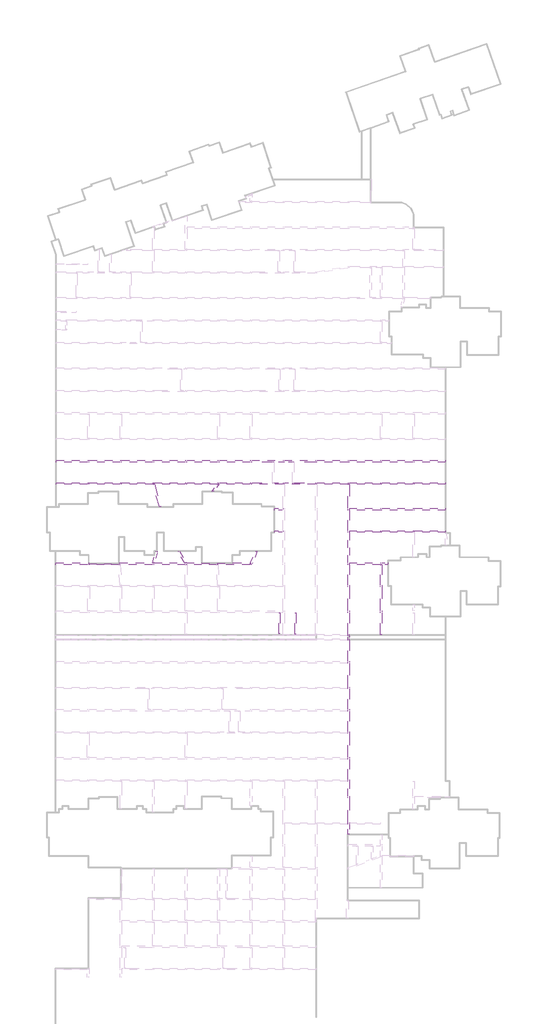
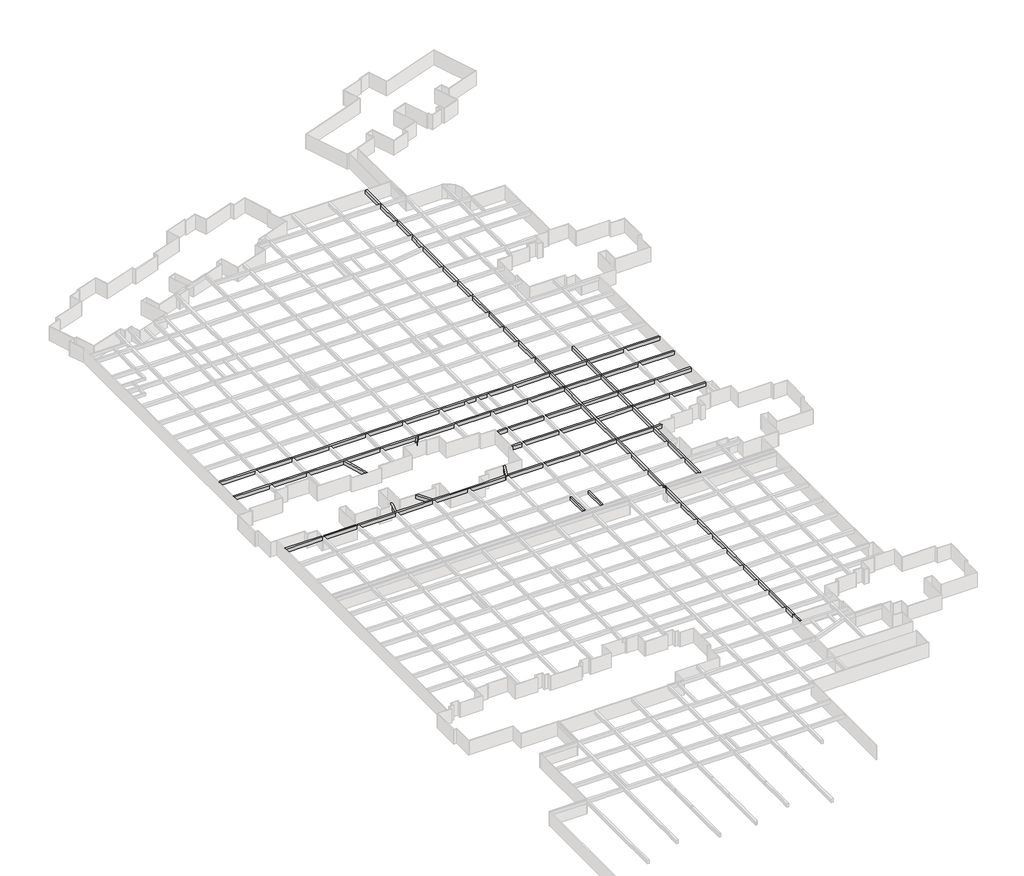
# One storey, part 11 of 14: 17 beams.
"""IFC4 building model written with IfcOpenShell, lengths in millimetres."""

from ifc_helpers import new_model, si_unit, frame, origin, place, context, project, spatial, polyline, outline, extrude, faceted_brep, element, save

model = new_model("IFC4")

# Units and contexts
model_context = context("Model", 3, world=origin())
ifc_project = project(units=[si_unit("LENGTHUNIT", "METRE", prefix="MILLI")], contexts=[model_context])

# Site, building, storey
site = spatial("IfcSite", under=ifc_project)
building = spatial("IfcBuilding", under=site)
storey = spatial("IfcBuildingStorey", under=building, Name="户型图", Elevation=0.0)

# Beams
placement = place(None, origin())
element("IfcBeam", 1, ObjectType="混凝土 - 矩形梁 : KL_beam", at=placement, inside=storey, context=model_context, shape_type="Brep", body=[
    faceted_brep([(-594019.2557706, -85259.4327531, 3300.0), (-594019.2557706, -85659.4327531, 3300.0), (-586267.6529954, -85659.4327531, 3300.0), (-585867.6529954, -85659.4327531, 3300.0), (-578267.6529954, -85659.4327531, 3300.0), (-577867.6529954, -85659.4327531, 3300.0), (-570267.6529954, -85659.4327531, 3300.0), (-569867.6529954, -85659.4327531, 3300.0), (-562267.6529954, -85659.4327531, 3300.0), (-561867.6529954, -85659.4327531, 3300.0), (-554267.6529954, -85659.4327531, 3300.0), (-553867.6529954, -85659.4327531, 3300.0), (-546267.6529954, -85659.4327531, 3300.0), (-545867.6529954, -85659.4327531, 3300.0), (-540767.6529954, -85659.4327531, 3300.0), (-540467.6529954, -85659.4327531, 3300.0), (-538267.6529954, -85659.4327531, 3300.0), (-537867.6529954, -85659.4327531, 3300.0), (-535867.6529954, -85659.4327531, 3300.0), (-535567.6529954, -85659.4327531, 3300.0), (-530267.6529954, -85659.4327531, 3300.0), (-529867.6529954, -85659.4327531, 3300.0), (-522267.6529954, -85659.4327531, 3300.0), (-521867.6529954, -85659.4327531, 3300.0), (-514267.6529954, -85659.4327531, 3300.0), (-513867.6529954, -85659.4327531, 3300.0), (-506267.6529954, -85659.4327531, 3300.0), (-505867.6529954, -85659.4327531, 3300.0), (-498277.6529954, -85659.4327531, 3300.0), (-498277.6529954, -85259.4327531, 3300.0), (-505867.6529954, -85259.4327531, 3300.0), (-506267.6529954, -85259.4327531, 3300.0), (-513867.6529954, -85259.4327531, 3300.0), (-514267.6529954, -85259.4327531, 3300.0), (-521867.6529954, -85259.4327531, 3300.0), (-522267.6529954, -85259.4327531, 3300.0), (-529867.6529954, -85259.4327531, 3300.0), (-530267.6529954, -85259.4327531, 3300.0), (-537867.6529954, -85259.4327531, 3300.0), (-538267.6529954, -85259.4327531, 3300.0), (-545867.6529954, -85259.4327531, 3300.0), (-546267.6529954, -85259.4327531, 3300.0), (-553867.6529954, -85259.4327531, 3300.0), (-554267.6529954, -85259.4327531, 3300.0), (-561867.6529954, -85259.4327531, 3300.0), (-562267.6529954, -85259.4327531, 3300.0), (-569867.6529954, -85259.4327531, 3300.0), (-570267.6529954, -85259.4327531, 3300.0), (-577867.6529954, -85259.4327531, 3300.0), (-578267.6529954, -85259.4327531, 3300.0), (-585867.6529954, -85259.4327531, 3300.0), (-586267.6529954, -85259.4327531, 3300.0), (-594019.2557706, -85659.4327531, 2500.0), (-586267.6529954, -85659.4327531, 2500.0), (-585867.6529954, -85659.4327531, 2500.0), (-578267.6529954, -85659.4327531, 2500.0), (-577867.6529954, -85659.4327531, 2500.0), (-570267.6529954, -85659.4327531, 2500.0), (-569867.6529954, -85659.4327531, 2500.0), (-562267.6529954, -85659.4327531, 2500.0), (-561867.6529954, -85659.4327531, 2500.0), (-554267.6529954, -85659.4327531, 2500.0), (-553867.6529954, -85659.4327531, 2500.0), (-546267.6529954, -85659.4327531, 2500.0), (-545867.6529954, -85659.4327531, 2500.0), (-538267.6529954, -85659.4327531, 2500.0), (-537867.6529954, -85659.4327531, 2500.0), (-530267.6529954, -85659.4327531, 2500.0), (-529867.6529954, -85659.4327531, 2500.0), (-522267.6529954, -85659.4327531, 2500.0), (-521867.6529954, -85659.4327531, 2500.0), (-514267.6529954, -85659.4327531, 2500.0), (-513867.6529954, -85659.4327531, 2500.0), (-506267.6529954, -85659.4327531, 2500.0), (-505867.6529954, -85659.4327531, 2500.0), (-498277.6529954, -85659.4327531, 2500.0), (-594019.2557706, -85259.4327531, 2500.0), (-586267.6529954, -85259.4327531, 2500.0), (-585867.6529954, -85259.4327531, 2500.0), (-578267.6529954, -85259.4327531, 2500.0), (-577867.6529954, -85259.4327531, 2500.0), (-570267.6529954, -85259.4327531, 2500.0), (-569867.6529954, -85259.4327531, 2500.0), (-562267.6529954, -85259.4327531, 2500.0), (-561867.6529954, -85259.4327531, 2500.0), (-554267.6529954, -85259.4327531, 2500.0), (-553867.6529954, -85259.4327531, 2500.0), (-546267.6529954, -85259.4327531, 2500.0), (-545867.6529954, -85259.4327531, 2500.0), (-538267.6529954, -85259.4327531, 2500.0), (-537867.6529954, -85259.4327531, 2500.0), (-530267.6529954, -85259.4327531, 2500.0), (-529867.6529954, -85259.4327531, 2500.0), (-522267.6529954, -85259.4327531, 2500.0), (-521867.6529954, -85259.4327531, 2500.0), (-514267.6529954, -85259.4327531, 2500.0), (-513867.6529954, -85259.4327531, 2500.0), (-506267.6529954, -85259.4327531, 2500.0), (-505867.6529954, -85259.4327531, 2500.0), (-498277.6529954, -85259.4327531, 2500.0)], [[[0, 1, 2, 3, 4, 5, 6, 7, 8, 9, 10, 11, 12, 13, 14, 15, 16, 17, 18, 19, 20, 21, 22, 23, 24, 25, 26, 27, 28, 29, 30, 31, 32, 33, 34, 35, 36, 37, 38, 39, 40, 41, 42, 43, 44, 45, 46, 47, 48, 49, 50, 51]], [[1, 52, 53, 54, 55, 56, 57, 58, 59, 60, 61, 62, 63, 64, 65, 66, 67, 68, 69, 70, 71, 72, 73, 74, 75, 28, 27, 26, 25, 24, 23, 22, 21, 20, 19, 18, 17, 16, 15, 14, 13, 12, 11, 10, 9, 8, 7, 6, 5, 4, 3, 2]], [[52, 76, 77, 78, 79, 80, 81, 82, 83, 84, 85, 86, 87, 88, 89, 90, 91, 92, 93, 94, 95, 96, 97, 98, 99, 75, 74, 73, 72, 71, 70, 69, 68, 67, 66, 65, 64, 63, 62, 61, 60, 59, 58, 57, 56, 55, 54, 53]], [[76, 0, 51, 50, 49, 48, 47, 46, 45, 44, 43, 42, 41, 40, 39, 38, 37, 36, 35, 34, 33, 32, 31, 30, 29, 99, 98, 97, 96, 95, 94, 93, 92, 91, 90, 89, 88, 87, 86, 85, 84, 83, 82, 81, 80, 79, 78, 77]], [[1, 0, 76, 52]], [[29, 28, 75, 99]]]),
])
element("IfcBeam", 2, ObjectType="混凝土 - 矩形梁 : KL_beam", at=placement, inside=storey, context=model_context, shape_type="Brep", body=[
    faceted_brep([(-594019.2557706, -90759.4327531, 3300.0), (-594019.2557706, -91159.4327531, 3300.0), (-586267.6529954, -91159.4327531, 3300.0), (-585867.6529954, -91159.4327531, 3300.0), (-578267.6529954, -91159.4327531, 3300.0), (-577867.6529954, -91159.4327531, 3300.0), (-570217.8756354, -91159.4327531, 3300.0), (-569801.3815466, -91159.4327531, 3300.0), (-562267.6529954, -91159.4327531, 3300.0), (-561867.6529954, -91159.4327531, 3300.0), (-554452.1630717, -91159.4327531, 3300.0), (-553963.8532362, -91159.4327531, 3300.0), (-546267.6529954, -91159.4327531, 3300.0), (-545867.6529954, -91159.4327531, 3300.0), (-538267.6529954, -91159.4327531, 3300.0), (-537867.6529954, -91159.4327531, 3300.0), (-530267.6529954, -91159.4327531, 3300.0), (-529867.6529954, -91159.4327531, 3300.0), (-522267.6529954, -91159.4327531, 3300.0), (-521867.6529954, -91159.4327531, 3300.0), (-514267.6529954, -91159.4327531, 3300.0), (-513867.6529954, -91159.4327531, 3300.0), (-506267.6529954, -91159.4327531, 3300.0), (-505867.6529954, -91159.4327531, 3300.0), (-498277.6529954, -91159.4327531, 3300.0), (-498277.6529954, -90759.4327531, 3300.0), (-505867.6529954, -90759.4327531, 3300.0), (-506267.6529954, -90759.4327531, 3300.0), (-513867.6529954, -90759.4327531, 3300.0), (-514267.6529954, -90759.4327531, 3300.0), (-521867.6529954, -90759.4327531, 3300.0), (-522267.6529954, -90759.4327531, 3300.0), (-529867.6529954, -90759.4327531, 3300.0), (-530267.6529954, -90759.4327531, 3300.0), (-535567.6529954, -90759.4327531, 3300.0), (-535867.6529954, -90759.4327531, 3300.0), (-537867.6529954, -90759.4327531, 3300.0), (-538267.6529954, -90759.4327531, 3300.0), (-540467.6529954, -90759.4327531, 3300.0), (-540767.6529954, -90759.4327531, 3300.0), (-545867.6529954, -90759.4327531, 3300.0), (-546267.6529954, -90759.4327531, 3300.0), (-553867.6529954, -90759.4327531, 3300.0), (-554267.6529954, -90759.4327531, 3300.0), (-561867.6529954, -90759.4327531, 3300.0), (-562267.6529954, -90759.4327531, 3300.0), (-569867.6529954, -90759.4327531, 3300.0), (-570267.6529954, -90759.4327531, 3300.0), (-577867.6529954, -90759.4327531, 3300.0), (-578267.6529954, -90759.4327531, 3300.0), (-585867.6529954, -90759.4327531, 3300.0), (-586267.6529954, -90759.4327531, 3300.0), (-594019.2557706, -90759.4327531, 2500.0), (-498277.6529954, -90759.4327531, 2500.0), (-505867.6529954, -90759.4327531, 2500.0), (-506267.6529954, -90759.4327531, 2500.0), (-513867.6529954, -90759.4327531, 2500.0), (-514267.6529954, -90759.4327531, 2500.0), (-521867.6529954, -90759.4327531, 2500.0), (-522267.6529954, -90759.4327531, 2500.0), (-529867.6529954, -90759.4327531, 2500.0), (-530267.6529954, -90759.4327531, 2500.0), (-537867.6529954, -90759.4327531, 2500.0), (-538267.6529954, -90759.4327531, 2500.0), (-545867.6529954, -90759.4327531, 2500.0), (-546267.6529954, -90759.4327531, 2500.0), (-553867.6529954, -90759.4327531, 2500.0), (-554267.6529954, -90759.4327531, 2500.0), (-561867.6529954, -90759.4327531, 2500.0), (-562267.6529954, -90759.4327531, 2500.0), (-569867.6529954, -90759.4327531, 2500.0), (-570267.6529954, -90759.4327531, 2500.0), (-577867.6529954, -90759.4327531, 2500.0), (-578267.6529954, -90759.4327531, 2500.0), (-585867.6529954, -90759.4327531, 2500.0), (-586267.6529954, -90759.4327531, 2500.0), (-594019.2557706, -91159.4327531, 2500.0), (-498277.6529954, -91159.4327531, 2500.0), (-505867.6529954, -91159.4327531, 2500.0), (-506267.6529954, -91159.4327531, 2500.0), (-513867.6529954, -91159.4327531, 2500.0), (-514267.6529954, -91159.4327531, 2500.0), (-521867.6529954, -91159.4327531, 2500.0), (-522267.6529954, -91159.4327531, 2500.0), (-529867.6529954, -91159.4327531, 2500.0), (-530267.6529954, -91159.4327531, 2500.0), (-537867.6529954, -91159.4327531, 2500.0), (-538267.6529954, -91159.4327531, 2500.0), (-545867.6529954, -91159.4327531, 2500.0), (-546267.6529954, -91159.4327531, 2500.0), (-553963.8532362, -91159.4327531, 2500.0), (-554452.1630717, -91159.4327531, 2500.0), (-561867.6529954, -91159.4327531, 2500.0), (-562267.6529954, -91159.4327531, 2500.0), (-569801.3815466, -91159.4327531, 2500.0), (-570217.8756354, -91159.4327531, 2500.0), (-577867.6529954, -91159.4327531, 2500.0), (-578267.6529954, -91159.4327531, 2500.0), (-585867.6529954, -91159.4327531, 2500.0), (-586267.6529954, -91159.4327531, 2500.0)], [[[0, 1, 2, 3, 4, 5, 6, 7, 8, 9, 10, 11, 12, 13, 14, 15, 16, 17, 18, 19, 20, 21, 22, 23, 24, 25, 26, 27, 28, 29, 30, 31, 32, 33, 34, 35, 36, 37, 38, 39, 40, 41, 42, 43, 44, 45, 46, 47, 48, 49, 50, 51]], [[52, 0, 51, 50, 49, 48, 47, 46, 45, 44, 43, 42, 41, 40, 39, 38, 37, 36, 35, 34, 33, 32, 31, 30, 29, 28, 27, 26, 25, 53, 54, 55, 56, 57, 58, 59, 60, 61, 62, 63, 64, 65, 66, 67, 68, 69, 70, 71, 72, 73, 74, 75]], [[76, 52, 75, 74, 73, 72, 71, 70, 69, 68, 67, 66, 65, 64, 63, 62, 61, 60, 59, 58, 57, 56, 55, 54, 53, 77, 78, 79, 80, 81, 82, 83, 84, 85, 86, 87, 88, 89, 90, 91, 92, 93, 94, 95, 96, 97, 98, 99]], [[1, 76, 99, 98, 97, 96, 95, 94, 93, 92, 91, 90, 89, 88, 87, 86, 85, 84, 83, 82, 81, 80, 79, 78, 77, 24, 23, 22, 21, 20, 19, 18, 17, 16, 15, 14, 13, 12, 11, 10, 9, 8, 7, 6, 5, 4, 3, 2]], [[1, 0, 52, 76]], [[25, 24, 77, 53]]]),
])
element("IfcBeam", 3, ObjectType="混凝土 - 矩形梁 : KL_beam", at=placement, inside=storey, context=model_context, shape_type="SweptSolid", body=[
    extrude(outline(polyline([(-568206.7540557, -96655.8355445), (-568623.2481445, -96655.8355445), (-570217.8756354, -91159.4327531), (-569801.3815466, -91159.4327531), (-568206.7540557, -96655.8355445)])), frame((0.0, 0.0, 2500.0), z_axis=(0.0, 0.0, 1.0), x_axis=(1.0, 0.0, 0.0)), (0.0, 0.0, 1.0), 800.0),
])
element("IfcBeam", 4, ObjectType="混凝土 - 矩形梁 : KL_beam", at=placement, inside=storey, context=model_context, shape_type="Brep", body=[
    faceted_brep([(-521867.6529954, -16219.4327531, 3300.0), (-522267.6529954, -16219.4327531, 3300.0), (-522267.6529954, -21559.4327531, 3300.0), (-521867.6529954, -21559.4327531, 3300.0), (-522267.6529954, -16219.4327531, 2500.0), (-522267.6529954, -21559.4327531, 2500.0), (-521867.6529954, -16219.4327531, 2500.0), (-521867.6529954, -21559.4327531, 2500.0)], [[[0, 1, 2, 3]], [[1, 4, 5, 2]], [[4, 6, 7, 5]], [[6, 0, 3, 7]], [[1, 0, 6, 4]], [[3, 2, 5, 7]]]),
    faceted_brep([(-521867.6529954, -177127.2416788, 3300.0), (-522267.6529954, -177127.2416788, 3300.0), (-522267.6529954, -177127.2416788, 2500.0), (-521867.6529954, -177127.2416788, 2500.0), (-522267.6529954, -91159.4327531, 3300.0), (-521867.6529954, -91159.4327531, 3300.0), (-521867.6529954, -91159.4327531, 2500.0), (-522267.6529954, -91159.4327531, 2500.0), (-521952.6098527, -128219.4327532, 2500.0), (-521952.6098527, -128219.4327532, 3300.0), (-521867.6529954, -128219.4327532, 3300.0), (-521867.6529954, -128219.4327532, 2500.0), (-521952.6098527, -128099.4327532, 3300.0), (-521952.6098527, -128099.4327532, 2500.0), (-521867.6529954, -128099.4327532, 2500.0), (-521867.6529954, -128099.4327532, 3300.0), (-521952.6098527, -129174.4327531, 3300.0), (-521952.6098527, -129174.4327531, 2500.0), (-521867.6529954, -129174.4327531, 2500.0), (-521867.6529954, -129174.4327531, 3300.0), (-521952.6098527, -129294.4327531, 2500.0), (-521952.6098527, -129294.4327531, 3300.0), (-521867.6529954, -129294.4327531, 3300.0), (-521867.6529954, -129294.4327531, 2500.0), (-521867.6529954, -174657.5200046, 3300.0), (-521867.6529954, -174257.5200046, 3300.0), (-521867.6529954, -168200.507479, 3300.0), (-521867.6529954, -167800.507479, 3300.0), (-521867.6529954, -164159.4327531, 3300.0), (-521867.6529954, -163759.4327531, 3300.0), (-521867.6529954, -158659.4327531, 3300.0), (-521867.6529954, -158259.4327531, 3300.0), (-521867.6529954, -152359.4327531, 3300.0), (-521867.6529954, -151959.4327531, 3300.0), (-521867.6529954, -146859.4327531, 3300.0), (-521867.6529954, -146459.4327531, 3300.0), (-521867.6529954, -141359.4327531, 3300.0), (-521867.6529954, -140959.4327531, 3300.0), (-521867.6529954, -135059.4327531, 3300.0), (-521867.6529954, -134659.4327531, 3300.0), (-521867.6529954, -129434.4327531, 3300.0), (-521867.6529954, -129034.4327531, 3300.0), (-521867.6529954, -128359.4327532, 3300.0), (-521867.6529954, -127959.4327532, 3300.0), (-521867.6529954, -122659.4327531, 3300.0), (-521867.6529954, -122259.4327531, 3300.0), (-521867.6529954, -116357.5126628, 3300.0), (-521867.6529954, -115957.5126628, 3300.0), (-521867.6529954, -110859.4327531, 3300.0), (-521867.6529954, -110459.4327531, 3300.0), (-521867.6529954, -102959.4327531, 3300.0), (-521867.6529954, -102559.4327531, 3300.0), (-521867.6529954, -97459.4327531, 3300.0), (-521867.6529954, -97059.4327531, 3300.0), (-522267.6529954, -97059.4327531, 3300.0), (-522267.6529954, -97459.4327531, 3300.0), (-522267.6529954, -102559.4327531, 3300.0), (-522267.6529954, -102959.4327531, 3300.0), (-522267.6529954, -110459.4327531, 3300.0), (-522267.6529954, -110859.4327531, 3300.0), (-522267.6529954, -115957.5126628, 3300.0), (-522267.6529954, -116357.5126628, 3300.0), (-522267.6529954, -122259.4327531, 3300.0), (-522267.6529954, -122659.4327531, 3300.0), (-522267.6529954, -127959.4327532, 3300.0), (-522267.6529954, -128359.4327532, 3300.0), (-522267.6529954, -129034.4327531, 3300.0), (-522267.6529954, -129434.4327531, 3300.0), (-522267.6529954, -134659.4327531, 3300.0), (-522267.6529954, -135059.4327531, 3300.0), (-522267.6529954, -140959.4327531, 3300.0), (-522267.6529954, -141359.4327531, 3300.0), (-522267.6529954, -146459.4327531, 3300.0), (-522267.6529954, -146859.4327531, 3300.0), (-522267.6529954, -151959.4327531, 3300.0), (-522267.6529954, -152359.4327531, 3300.0), (-522267.6529954, -158259.4327531, 3300.0), (-522267.6529954, -158659.4327531, 3300.0), (-522267.6529954, -163759.4327531, 3300.0), (-522267.6529954, -164159.4327531, 3300.0), (-522267.6529954, -167800.507479, 3300.0), (-522267.6529954, -168200.507479, 3300.0), (-522267.6529954, -174257.5200046, 3300.0), (-522267.6529954, -174657.5200046, 3300.0), (-522267.6529954, -97059.4327531, 2500.0), (-522267.6529954, -97459.4327531, 2500.0), (-522267.6529954, -102559.4327531, 2500.0), (-522267.6529954, -102959.4327531, 2500.0), (-522267.6529954, -110459.4327531, 2500.0), (-522267.6529954, -110859.4327531, 2500.0), (-522267.6529954, -115957.5126628, 2500.0), (-522267.6529954, -116357.5126628, 2500.0), (-522267.6529954, -122259.4327531, 2500.0), (-522267.6529954, -122659.4327531, 2500.0), (-522267.6529954, -127959.4327532, 2500.0), (-522267.6529954, -128359.4327532, 2500.0), (-522267.6529954, -129034.4327531, 2500.0), (-522267.6529954, -129434.4327531, 2500.0), (-522267.6529954, -134659.4327531, 2500.0), (-522267.6529954, -135059.4327531, 2500.0), (-522267.6529954, -140959.4327531, 2500.0), (-522267.6529954, -141359.4327531, 2500.0), (-522267.6529954, -146459.4327531, 2500.0), (-522267.6529954, -146859.4327531, 2500.0), (-522267.6529954, -151959.4327531, 2500.0), (-522267.6529954, -152359.4327531, 2500.0), (-522267.6529954, -158259.4327531, 2500.0), (-522267.6529954, -158659.4327531, 2500.0), (-522267.6529954, -163759.4327531, 2500.0), (-522267.6529954, -164159.4327531, 2500.0), (-522267.6529954, -167800.507479, 2500.0), (-522267.6529954, -168200.507479, 2500.0), (-522267.6529954, -174257.5200046, 2500.0), (-522267.6529954, -174657.5200046, 2500.0), (-521867.6529954, -97059.4327531, 2500.0), (-521867.6529954, -97459.4327531, 2500.0), (-521867.6529954, -102559.4327531, 2500.0), (-521867.6529954, -102959.4327531, 2500.0), (-521867.6529954, -110459.4327531, 2500.0), (-521867.6529954, -110859.4327531, 2500.0), (-521867.6529954, -115957.5126628, 2500.0), (-521867.6529954, -116357.5126628, 2500.0), (-521867.6529954, -122259.4327531, 2500.0), (-521867.6529954, -122659.4327531, 2500.0), (-521867.6529954, -127959.4327532, 2500.0), (-521867.6529954, -128359.4327532, 2500.0), (-521867.6529954, -129034.4327531, 2500.0), (-521867.6529954, -129434.4327531, 2500.0), (-521867.6529954, -134659.4327531, 2500.0), (-521867.6529954, -135059.4327531, 2500.0), (-521867.6529954, -140959.4327531, 2500.0), (-521867.6529954, -141359.4327531, 2500.0), (-521867.6529954, -146459.4327531, 2500.0), (-521867.6529954, -146859.4327531, 2500.0), (-521867.6529954, -151959.4327531, 2500.0), (-521867.6529954, -152359.4327531, 2500.0), (-521867.6529954, -158259.4327531, 2500.0), (-521867.6529954, -158659.4327531, 2500.0), (-521867.6529954, -163759.4327531, 2500.0), (-521867.6529954, -164159.4327531, 2500.0), (-521867.6529954, -167800.507479, 2500.0), (-521867.6529954, -168200.507479, 2500.0), (-521867.6529954, -174257.5200046, 2500.0), (-521867.6529954, -174657.5200046, 2500.0)], [[[0, 1, 2, 3]], [[4, 5, 6, 7]], [[8, 9, 10, 11]], [[12, 13, 14, 15]], [[9, 8, 13, 12]], [[16, 17, 18, 19]], [[20, 21, 22, 23]], [[17, 16, 21, 20]], [[1, 0, 24, 25, 26, 27, 28, 29, 30, 31, 32, 33, 34, 35, 36, 37, 38, 39, 40, 22, 21, 16, 19, 41, 42, 10, 9, 12, 15, 43, 44, 45, 46, 47, 48, 49, 50, 51, 52, 53, 5, 4, 54, 55, 56, 57, 58, 59, 60, 61, 62, 63, 64, 65, 66, 67, 68, 69, 70, 71, 72, 73, 74, 75, 76, 77, 78, 79, 80, 81, 82, 83]], [[2, 1, 83, 82, 81, 80, 79, 78, 77, 76, 75, 74, 73, 72, 71, 70, 69, 68, 67, 66, 65, 64, 63, 62, 61, 60, 59, 58, 57, 56, 55, 54, 4, 7, 84, 85, 86, 87, 88, 89, 90, 91, 92, 93, 94, 95, 96, 97, 98, 99, 100, 101, 102, 103, 104, 105, 106, 107, 108, 109, 110, 111, 112, 113]], [[3, 2, 113, 112, 111, 110, 109, 108, 107, 106, 105, 104, 103, 102, 101, 100, 99, 98, 97, 96, 95, 94, 93, 92, 91, 90, 89, 88, 87, 86, 85, 84, 7, 6, 114, 115, 116, 117, 118, 119, 120, 121, 122, 123, 124, 14, 13, 8, 11, 125, 126, 18, 17, 20, 23, 127, 128, 129, 130, 131, 132, 133, 134, 135, 136, 137, 138, 139, 140, 141, 142, 143]], [[0, 3, 143, 142, 141, 140, 139, 138, 137, 136, 135, 134, 133, 132, 131, 130, 129, 128, 127, 23, 22, 40, 39, 38, 37, 36, 35, 34, 33, 32, 31, 30, 29, 28, 27, 26, 25, 24]], [[6, 5, 53, 52, 51, 50, 49, 48, 47, 46, 45, 44, 43, 15, 14, 124, 123, 122, 121, 120, 119, 118, 117, 116, 115, 114]], [[11, 10, 42, 41, 19, 18, 126, 125]]]),
    faceted_brep([(-522267.6529954, -33759.4327531, 3300.0), (-521867.6529954, -33759.4327531, 3300.0), (-521867.6529954, -33759.4327531, 2500.0), (-522267.6529954, -33759.4327531, 2500.0), (-521867.6529954, -45159.4327531, 3300.0), (-522267.6529954, -45159.4327531, 3300.0), (-522267.6529954, -45159.4327531, 2500.0), (-521867.6529954, -45159.4327531, 2500.0), (-522267.6529954, -37589.309334, 3300.0), (-522267.6529954, -37994.5561723, 3300.0), (-521867.6529954, -37959.4327532, 3300.0), (-521867.6529954, -37559.4327532, 3300.0), (-522267.6529954, -37589.309334, 2500.0), (-522267.6529954, -37994.5561723, 2500.0), (-521867.6529954, -37559.4327532, 2500.0), (-521867.6529954, -37959.4327532, 2500.0)], [[[0, 1, 2, 3]], [[4, 5, 6, 7]], [[1, 0, 8, 9, 5, 4, 10, 11]], [[0, 3, 12, 13, 6, 5, 9, 8]], [[3, 2, 14, 15, 7, 6, 13, 12]], [[2, 1, 11, 10, 4, 7, 15, 14]]]),
    faceted_brep([(-521867.6529954, -33359.4327531, 3300.0), (-522267.6529954, -33359.4327531, 3300.0), (-522267.6529954, -33359.4327531, 2500.0), (-521867.6529954, -33359.4327531, 2500.0), (-522267.6529954, -28259.4327531, 3300.0), (-521867.6529954, -28259.4327531, 3300.0), (-521867.6529954, -28259.4327531, 2500.0), (-522267.6529954, -28259.4327531, 2500.0)], [[[0, 1, 2, 3]], [[4, 5, 6, 7]], [[1, 0, 5, 4]], [[2, 1, 4, 7]], [[3, 2, 7, 6]], [[0, 3, 6, 5]]]),
    faceted_brep([(-521867.6529954, -27859.4327531, 3300.0), (-522267.6529954, -27859.4327531, 3300.0), (-522267.6529954, -27859.4327531, 2500.0), (-521867.6529954, -27859.4327531, 2500.0), (-522267.6529954, -21959.4327531, 3300.0), (-521867.6529954, -21959.4327531, 3300.0), (-521867.6529954, -21959.4327531, 2500.0), (-522267.6529954, -21959.4327531, 2500.0)], [[[0, 1, 2, 3]], [[4, 5, 6, 7]], [[1, 0, 5, 4]], [[2, 1, 4, 7]], [[3, 2, 7, 6]], [[0, 3, 6, 5]]]),
    faceted_brep([(-522267.6529954, -45559.4327531, 3300.0), (-521867.6529954, -45559.4327531, 3300.0), (-521867.6529954, -45559.4327531, 2500.0), (-522267.6529954, -45559.4327531, 2500.0), (-521867.6529954, -50659.4327531, 3300.0), (-522267.6529954, -50659.4327531, 3300.0), (-522267.6529954, -50659.4327531, 2500.0), (-521867.6529954, -50659.4327531, 2500.0)], [[[0, 1, 2, 3]], [[4, 5, 6, 7]], [[1, 0, 5, 4]], [[0, 3, 6, 5]], [[3, 2, 7, 6]], [[2, 1, 4, 7]]]),
    faceted_brep([(-522267.6529954, -56559.4327531, 3300.0), (-521867.6529954, -56559.4327531, 3300.0), (-521867.6529954, -56559.4327531, 2500.0), (-522267.6529954, -56559.4327531, 2500.0), (-521867.6529954, -62459.4327531, 3300.0), (-522267.6529954, -62459.4327531, 3300.0), (-522267.6529954, -62459.4327531, 2500.0), (-521867.6529954, -62459.4327531, 2500.0)], [[[0, 1, 2, 3]], [[4, 5, 6, 7]], [[1, 0, 5, 4]], [[0, 3, 6, 5]], [[3, 2, 7, 6]], [[2, 1, 4, 7]]]),
    faceted_brep([(-521867.6529954, -56159.4327531, 3300.0), (-522267.6529954, -56159.4327531, 3300.0), (-522267.6529954, -56159.4327531, 2500.0), (-521867.6529954, -56159.4327531, 2500.0), (-522267.6529954, -51059.4327531, 3300.0), (-521867.6529954, -51059.4327531, 3300.0), (-521867.6529954, -51059.4327531, 2500.0), (-522267.6529954, -51059.4327531, 2500.0)], [[[0, 1, 2, 3]], [[4, 5, 6, 7]], [[1, 0, 5, 4]], [[2, 1, 4, 7]], [[3, 2, 7, 6]], [[0, 3, 6, 5]]]),
    faceted_brep([(-522267.6529954, -62859.4327531, 3300.0), (-521867.6529954, -62859.4327531, 3300.0), (-521867.6529954, -62859.4327531, 2500.0), (-522267.6529954, -62859.4327531, 2500.0), (-521867.6529954, -67959.4327531, 3300.0), (-522267.6529954, -67959.4327531, 3300.0), (-522267.6529954, -67959.4327531, 2500.0), (-521867.6529954, -67959.4327531, 2500.0)], [[[0, 1, 2, 3]], [[4, 5, 6, 7]], [[1, 0, 5, 4]], [[0, 3, 6, 5]], [[3, 2, 7, 6]], [[2, 1, 4, 7]]]),
    faceted_brep([(-522267.6529954, -68359.4327531, 3300.0), (-521867.6529954, -68359.4327531, 3300.0), (-521867.6529954, -68359.4327531, 2500.0), (-522267.6529954, -68359.4327531, 2500.0), (-521867.6529954, -73459.4327531, 3300.0), (-522267.6529954, -73459.4327531, 3300.0), (-522267.6529954, -73459.4327531, 2500.0), (-521867.6529954, -73459.4327531, 2500.0)], [[[0, 1, 2, 3]], [[4, 5, 6, 7]], [[1, 0, 5, 4]], [[0, 3, 6, 5]], [[3, 2, 7, 6]], [[2, 1, 4, 7]]]),
    faceted_brep([(-522267.6529954, -73859.4327531, 3300.0), (-521867.6529954, -73859.4327531, 3300.0), (-521867.6529954, -73859.4327531, 2500.0), (-522267.6529954, -73859.4327531, 2500.0), (-521867.6529954, -79759.4327531, 3300.0), (-522267.6529954, -79759.4327531, 3300.0), (-522267.6529954, -79759.4327531, 2500.0), (-521867.6529954, -79759.4327531, 2500.0)], [[[0, 1, 2, 3]], [[4, 5, 6, 7]], [[1, 0, 5, 4]], [[0, 3, 6, 5]], [[3, 2, 7, 6]], [[2, 1, 4, 7]]]),
    faceted_brep([(-522267.6529954, -80159.4327531, 3300.0), (-521867.6529954, -80159.4327531, 3300.0), (-521867.6529954, -80159.4327531, 2500.0), (-522267.6529954, -80159.4327531, 2500.0), (-521867.6529954, -85259.4327531, 3300.0), (-522267.6529954, -85259.4327531, 3300.0), (-522267.6529954, -85259.4327531, 2500.0), (-521867.6529954, -85259.4327531, 2500.0)], [[[0, 1, 2, 3]], [[4, 5, 6, 7]], [[1, 0, 5, 4]], [[0, 3, 6, 5]], [[3, 2, 7, 6]], [[2, 1, 4, 7]]]),
    faceted_brep([(-522267.6529954, -85659.4327531, 3300.0), (-521867.6529954, -85659.4327531, 3300.0), (-521867.6529954, -85659.4327531, 2500.0), (-522267.6529954, -85659.4327531, 2500.0), (-521867.6529954, -90759.4327531, 3300.0), (-522267.6529954, -90759.4327531, 3300.0), (-522267.6529954, -90759.4327531, 2500.0), (-521867.6529954, -90759.4327531, 2500.0)], [[[0, 1, 2, 3]], [[4, 5, 6, 7]], [[1, 0, 5, 4]], [[0, 3, 6, 5]], [[3, 2, 7, 6]], [[2, 1, 4, 7]]]),
    faceted_brep([(-521867.6529954, -177247.2416788, 3300.0), (-521867.6529954, -177247.2416788, 2500.0), (-522183.9222774, -177247.2416788, 2500.0), (-522183.9222774, -177247.2416788, 3300.0), (-521867.6529954, -179652.8565433, 3300.0), (-522183.9222774, -179652.8565433, 3300.0), (-521867.6529954, -179652.8565433, 2500.0), (-522183.9222774, -179652.8565433, 2500.0)], [[[0, 1, 2, 3]], [[4, 0, 3, 5]], [[1, 6, 7, 2]], [[1, 0, 4, 6]], [[6, 4, 5, 7]], [[3, 2, 7, 5]]]),
])
element("IfcBeam", 5, ObjectType="混凝土 - 矩形梁 : KL_beam", at=placement, inside=storey, context=model_context, shape_type="SweptSolid", body=[
    extrude(outline(polyline([(-555116.6769089, -92805.8355834), (-555604.9867444, -92805.8355834), (-554452.1630717, -91159.4327531), (-553963.8532362, -91159.4327531), (-555116.6769089, -92805.8355834)])), frame((0.0, 0.0, 2500.0), z_axis=(0.0, 0.0, 1.0), x_axis=(1.0, 0.0, 0.0)), (0.0, 0.0, 1.0), 800.0),
])
element("IfcBeam", 6, ObjectType="混凝土 - 矩形梁 : KL_beam", at=placement, inside=storey, context=model_context, shape_type="SweptSolid", body=[
    extrude(outline(polyline([(-540337.593755, -97459.4327531), (-540337.593755, -97059.4327531), (-538267.6529954, -97059.4327531), (-538267.6529954, -97459.4327531), (-540337.593755, -97459.4327531)])), frame((0.0, 0.0, 2500.0), z_axis=(0.0, 0.0, 1.0), x_axis=(1.0, 0.0, 0.0)), (0.0, 0.0, 1.0), 800.0),
])
element("IfcBeam", 7, ObjectType="混凝土 - 矩形梁 : KL_beam", at=placement, inside=storey, context=model_context, shape_type="Brep", body=[
    faceted_brep([(-540337.593755, -102559.4327531, 3300.0), (-540337.593755, -102955.8355437, 3300.0), (-540337.593755, -102959.4327531, 3300.0), (-538267.6529954, -102959.4327531, 3300.0), (-538267.6529954, -102559.4327531, 3300.0), (-540337.593755, -102559.4327531, 2500.0), (-538267.6529954, -102559.4327531, 2500.0), (-540337.593755, -102959.4327531, 2500.0), (-538267.6529954, -102959.4327531, 2500.0)], [[[0, 1, 2, 3, 4]], [[5, 0, 4, 6]], [[7, 5, 6, 8]], [[8, 3, 2, 7]], [[0, 5, 7, 2, 1]], [[4, 3, 8, 6]]]),
])
element("IfcBeam", 8, ObjectType="混凝土 - 矩形梁 : KL_beam", at=placement, inside=storey, context=model_context, shape_type="Brep", body=[
    faceted_brep([(-537867.6529954, -97059.4327531, 3300.0), (-537867.6529954, -97459.4327531, 3300.0), (-530267.6529954, -97459.4327531, 3300.0), (-530267.6529954, -97059.4327531, 3300.0), (-537867.6529954, -97459.4327531, 2500.0), (-530267.6529954, -97459.4327531, 2500.0), (-537867.6529954, -97059.4327531, 2500.0), (-530267.6529954, -97059.4327531, 2500.0)], [[[0, 1, 2, 3]], [[1, 4, 5, 2]], [[4, 6, 7, 5]], [[6, 0, 3, 7]], [[1, 0, 6, 4]], [[3, 2, 5, 7]]]),
    faceted_brep([(-498277.6529954, -97059.4327531, 3300.0), (-498277.6529954, -97459.4327531, 3300.0), (-498277.6529954, -97459.4327531, 2500.0), (-498277.6529954, -97059.4327531, 2500.0), (-505867.6529954, -97059.4327531, 3300.0), (-506267.6529954, -97059.4327531, 3300.0), (-513867.6529954, -97059.4327531, 3300.0), (-514267.6529954, -97059.4327531, 3300.0), (-521867.6529954, -97059.4327531, 3300.0), (-521867.6529954, -97459.4327531, 3300.0), (-514267.6529954, -97459.4327531, 3300.0), (-513867.6529954, -97459.4327531, 3300.0), (-506267.6529954, -97459.4327531, 3300.0), (-505867.6529954, -97459.4327531, 3300.0), (-521867.6529954, -97459.4327531, 2500.0), (-514267.6529954, -97459.4327531, 2500.0), (-513867.6529954, -97459.4327531, 2500.0), (-506267.6529954, -97459.4327531, 2500.0), (-505867.6529954, -97459.4327531, 2500.0), (-521867.6529954, -97059.4327531, 2500.0), (-514267.6529954, -97059.4327531, 2500.0), (-513867.6529954, -97059.4327531, 2500.0), (-506267.6529954, -97059.4327531, 2500.0), (-505867.6529954, -97059.4327531, 2500.0)], [[[0, 1, 2, 3]], [[1, 0, 4, 5, 6, 7, 8, 9, 10, 11, 12, 13]], [[2, 1, 13, 12, 11, 10, 9, 14, 15, 16, 17, 18]], [[3, 2, 18, 17, 16, 15, 14, 19, 20, 21, 22, 23]], [[0, 3, 23, 22, 21, 20, 19, 8, 7, 6, 5, 4]], [[9, 8, 19, 14]]]),
    faceted_brep([(-529867.6529954, -97459.4327531, 3300.0), (-529867.6529954, -97059.4327531, 3300.0), (-529867.6529954, -97059.4327531, 2500.0), (-529867.6529954, -97459.4327531, 2500.0), (-522267.6529954, -97059.4327531, 3300.0), (-522267.6529954, -97459.4327531, 3300.0), (-522267.6529954, -97459.4327531, 2500.0), (-522267.6529954, -97059.4327531, 2500.0)], [[[0, 1, 2, 3]], [[4, 5, 6, 7]], [[1, 0, 5, 4]], [[0, 3, 6, 5]], [[3, 2, 7, 6]], [[2, 1, 4, 7]]]),
])
element("IfcBeam", 9, ObjectType="混凝土 - 矩形梁 : KL_beam", at=placement, inside=storey, context=model_context, shape_type="Brep", body=[
    faceted_brep([(-537867.6529954, -102559.4327531, 3300.0), (-537867.6529954, -102959.4327531, 3300.0), (-530267.6529954, -102959.4327531, 3300.0), (-530267.6529954, -102559.4327531, 3300.0), (-537867.6529954, -102959.4327531, 2500.0), (-530267.6529954, -102959.4327531, 2500.0), (-537867.6529954, -102559.4327531, 2500.0), (-530267.6529954, -102559.4327531, 2500.0)], [[[0, 1, 2, 3]], [[1, 4, 5, 2]], [[4, 6, 7, 5]], [[6, 0, 3, 7]], [[1, 0, 6, 4]], [[3, 2, 5, 7]]]),
    faceted_brep([(-498277.6529954, -102559.4327531, 3300.0), (-498277.6529954, -102959.4327531, 3300.0), (-498277.6529954, -102959.4327531, 2500.0), (-498277.6529954, -102559.4327531, 2500.0), (-505867.6529954, -102559.4327531, 3300.0), (-506267.6529954, -102559.4327531, 3300.0), (-513867.6529954, -102559.4327531, 3300.0), (-514267.6529954, -102559.4327531, 3300.0), (-521867.6529954, -102559.4327531, 3300.0), (-521867.6529954, -102959.4327531, 3300.0), (-514267.6529954, -102959.4327531, 3300.0), (-513867.6529954, -102959.4327531, 3300.0), (-506267.6529954, -102959.4327531, 3300.0), (-505867.6529954, -102959.4327531, 3300.0), (-521867.6529954, -102959.4327531, 2500.0), (-514267.6529954, -102959.4327531, 2500.0), (-513867.6529954, -102959.4327531, 2500.0), (-506267.6529954, -102959.4327531, 2500.0), (-505867.6529954, -102959.4327531, 2500.0), (-521867.6529954, -102559.4327531, 2500.0), (-514267.6529954, -102559.4327531, 2500.0), (-513867.6529954, -102559.4327531, 2500.0), (-506267.6529954, -102559.4327531, 2500.0), (-505867.6529954, -102559.4327531, 2500.0)], [[[0, 1, 2, 3]], [[1, 0, 4, 5, 6, 7, 8, 9, 10, 11, 12, 13]], [[2, 1, 13, 12, 11, 10, 9, 14, 15, 16, 17, 18]], [[3, 2, 18, 17, 16, 15, 14, 19, 20, 21, 22, 23]], [[0, 3, 23, 22, 21, 20, 19, 8, 7, 6, 5, 4]], [[9, 8, 19, 14]]]),
    faceted_brep([(-529867.6529954, -102959.4327531, 3300.0), (-529867.6529954, -102559.4327531, 3300.0), (-529867.6529954, -102559.4327531, 2500.0), (-529867.6529954, -102959.4327531, 2500.0), (-522267.6529954, -102559.4327531, 3300.0), (-522267.6529954, -102959.4327531, 3300.0), (-522267.6529954, -102959.4327531, 2500.0), (-522267.6529954, -102559.4327531, 2500.0)], [[[0, 1, 2, 3]], [[4, 5, 6, 7]], [[1, 0, 5, 4]], [[0, 3, 6, 5]], [[3, 2, 7, 6]], [[2, 1, 4, 7]]]),
])
element("IfcBeam", 10, ObjectType="混凝土 - 矩形梁 : KL_beam", at=placement, inside=storey, context=model_context, shape_type="Brep", body=[
    faceted_brep([(-546303.4778246, -110703.1403018, 3300.0), (-545935.2758832, -110859.4327531, 3300.0), (-545765.4859567, -110459.4327531, 3300.0), (-544541.4715612, -107575.8355437, 3300.0), (-544976.0157121, -107575.8355437, 3300.0), (-546200.0301077, -110459.4327531, 3300.0), (-545935.2758832, -110859.4327531, 2500.0), (-545765.4859567, -110459.4327531, 2500.0), (-544541.4715612, -107575.8355437, 2500.0), (-546303.4778246, -110703.1403018, 2500.0), (-546200.0301077, -110459.4327531, 2500.0), (-544976.0157121, -107575.8355437, 2500.0)], [[[0, 1, 2, 3, 4, 5]], [[1, 6, 7, 8, 3, 2]], [[6, 9, 10, 11, 8, 7]], [[9, 0, 5, 4, 11, 10]], [[4, 3, 8, 11]], [[0, 9, 6, 1]]]),
])
element("IfcBeam", 11, ObjectType="混凝土 - 矩形梁 : KL_beam", at=placement, inside=storey, context=model_context, shape_type="Brep", body=[
    faceted_brep([(-512410.8523761, -110859.4327531, 3300.0), (-512410.8523761, -110459.4327531, 3300.0), (-513867.6529954, -110459.4327531, 3300.0), (-514267.6529954, -110459.4327531, 3300.0), (-521867.6529954, -110459.4327531, 3300.0), (-521867.6529954, -110859.4327531, 3300.0), (-514267.6529954, -110859.4327531, 3300.0), (-513867.6529954, -110859.4327531, 3300.0), (-512410.8523761, -110859.4327531, 2500.0), (-521867.6529954, -110859.4327531, 2500.0), (-514267.6529954, -110859.4327531, 2500.0), (-513867.6529954, -110859.4327531, 2500.0), (-512410.8523761, -110459.4327531, 2500.0), (-521867.6529954, -110459.4327531, 2500.0), (-514267.6529954, -110459.4327531, 2500.0), (-513867.6529954, -110459.4327531, 2500.0)], [[[0, 1, 2, 3, 4, 5, 6, 7]], [[8, 0, 7, 6, 5, 9, 10, 11]], [[12, 8, 11, 10, 9, 13, 14, 15]], [[1, 12, 15, 14, 13, 4, 3, 2]], [[1, 0, 8, 12]], [[5, 4, 13, 9]]]),
    faceted_brep([(-545935.2758832, -110859.4327531, 3300.0), (-545765.4859567, -110459.4327531, 3300.0), (-545765.4859567, -110459.4327531, 2500.0), (-545935.2758832, -110859.4327531, 2500.0), (-538267.6529954, -110459.4327531, 3300.0), (-538267.6529954, -110859.4327531, 3300.0), (-538267.6529954, -110859.4327531, 2500.0), (-538267.6529954, -110459.4327531, 2500.0), (-545867.6529954, -110859.4327531, 3300.0), (-545867.6529954, -110859.4327531, 2500.0)], [[[0, 1, 2, 3]], [[4, 5, 6, 7]], [[1, 0, 8, 5, 4]], [[0, 3, 9, 6, 5, 8]], [[3, 2, 7, 6, 9]], [[2, 1, 4, 7]]]),
    faceted_brep([(-537867.6529954, -110859.4327531, 3300.0), (-537867.6529954, -110459.4327531, 3300.0), (-537867.6529954, -110459.4327531, 2500.0), (-537867.6529954, -110859.4327531, 2500.0), (-530267.6529954, -110459.4327531, 3300.0), (-530267.6529954, -110859.4327531, 3300.0), (-530267.6529954, -110859.4327531, 2500.0), (-530267.6529954, -110459.4327531, 2500.0)], [[[0, 1, 2, 3]], [[4, 5, 6, 7]], [[1, 0, 5, 4]], [[0, 3, 6, 5]], [[3, 2, 7, 6]], [[2, 1, 4, 7]]]),
    faceted_brep([(-529867.6529954, -110859.4327531, 3300.0), (-529867.6529954, -110459.4327531, 3300.0), (-529867.6529954, -110459.4327531, 2500.0), (-529867.6529954, -110859.4327531, 2500.0), (-522267.6529954, -110459.4327531, 3300.0), (-522267.6529954, -110859.4327531, 3300.0), (-522267.6529954, -110859.4327531, 2500.0), (-522267.6529954, -110459.4327531, 2500.0)], [[[0, 1, 2, 3]], [[4, 5, 6, 7]], [[1, 0, 5, 4]], [[0, 3, 6, 5]], [[3, 2, 7, 6]], [[2, 1, 4, 7]]]),
])
element("IfcBeam", 12, ObjectType="混凝土 - 矩形梁 : KL_beam", at=placement, inside=storey, context=model_context, shape_type="Brep", body=[
    faceted_brep([(-514267.6529954, -128099.4327532, 3300.0), (-513867.6529954, -128099.4327532, 3300.0), (-513867.6529954, -127959.4327532, 3300.0), (-513867.6529954, -122659.4327531, 3300.0), (-513867.6529954, -122259.4327531, 3300.0), (-513867.6529954, -116357.5126628, 3300.0), (-513867.6529954, -115957.5126628, 3300.0), (-513867.6529954, -110859.4327531, 3300.0), (-514267.6529954, -110859.4327531, 3300.0), (-514267.6529954, -115957.5126628, 3300.0), (-514267.6529954, -116357.5126628, 3300.0), (-514267.6529954, -122259.4327531, 3300.0), (-514267.6529954, -122659.4327531, 3300.0), (-514267.6529954, -127959.4327532, 3300.0), (-513867.6529954, -128099.4327532, 2500.0), (-513867.6529954, -127959.4327532, 2500.0), (-513867.6529954, -122659.4327531, 2500.0), (-513867.6529954, -122259.4327531, 2500.0), (-513867.6529954, -116357.5126628, 2500.0), (-513867.6529954, -115957.5126628, 2500.0), (-513867.6529954, -110859.4327531, 2500.0), (-514267.6529954, -128099.4327532, 2500.0), (-514267.6529954, -127959.4327532, 2500.0), (-514267.6529954, -122659.4327531, 2500.0), (-514267.6529954, -122259.4327531, 2500.0), (-514267.6529954, -116357.5126628, 2500.0), (-514267.6529954, -115957.5126628, 2500.0), (-514267.6529954, -110859.4327531, 2500.0)], [[[0, 1, 2, 3, 4, 5, 6, 7, 8, 9, 10, 11, 12, 13]], [[1, 14, 15, 16, 17, 18, 19, 20, 7, 6, 5, 4, 3, 2]], [[14, 21, 22, 23, 24, 25, 26, 27, 20, 19, 18, 17, 16, 15]], [[21, 0, 13, 12, 11, 10, 9, 8, 27, 26, 25, 24, 23, 22]], [[1, 0, 21, 14]], [[8, 7, 20, 27]]]),
    faceted_brep([(-514267.6529954, -80159.4327531, 3300.0), (-513867.6529954, -80159.4327531, 3300.0), (-513867.6529954, -80159.4327531, 2500.0), (-514267.6529954, -80159.4327531, 2500.0), (-513867.6529954, -85259.4327531, 3300.0), (-514267.6529954, -85259.4327531, 3300.0), (-514267.6529954, -85259.4327531, 2500.0), (-513867.6529954, -85259.4327531, 2500.0)], [[[0, 1, 2, 3]], [[4, 5, 6, 7]], [[1, 0, 5, 4]], [[2, 1, 4, 7]], [[3, 2, 7, 6]], [[0, 3, 6, 5]]]),
    faceted_brep([(-514267.6529954, -85659.4327531, 3300.0), (-513867.6529954, -85659.4327531, 3300.0), (-513867.6529954, -85659.4327531, 2500.0), (-514267.6529954, -85659.4327531, 2500.0), (-513867.6529954, -90759.4327531, 3300.0), (-514267.6529954, -90759.4327531, 3300.0), (-514267.6529954, -90759.4327531, 2500.0), (-513867.6529954, -90759.4327531, 2500.0)], [[[0, 1, 2, 3]], [[4, 5, 6, 7]], [[1, 0, 5, 4]], [[2, 1, 4, 7]], [[3, 2, 7, 6]], [[0, 3, 6, 5]]]),
    faceted_brep([(-514267.6529954, -91159.4327531, 3300.0), (-513867.6529954, -91159.4327531, 3300.0), (-513867.6529954, -91159.4327531, 2500.0), (-514267.6529954, -91159.4327531, 2500.0), (-513867.6529954, -97059.4327531, 3300.0), (-514267.6529954, -97059.4327531, 3300.0), (-514267.6529954, -97059.4327531, 2500.0), (-513867.6529954, -97059.4327531, 2500.0)], [[[0, 1, 2, 3]], [[4, 5, 6, 7]], [[1, 0, 5, 4]], [[2, 1, 4, 7]], [[3, 2, 7, 6]], [[0, 3, 6, 5]]]),
    faceted_brep([(-514267.6529954, -97459.4327531, 3300.0), (-513867.6529954, -97459.4327531, 3300.0), (-513867.6529954, -97459.4327531, 2500.0), (-514267.6529954, -97459.4327531, 2500.0), (-513867.6529954, -102559.4327531, 3300.0), (-514267.6529954, -102559.4327531, 3300.0), (-514267.6529954, -102559.4327531, 2500.0), (-513867.6529954, -102559.4327531, 2500.0)], [[[0, 1, 2, 3]], [[4, 5, 6, 7]], [[1, 0, 5, 4]], [[2, 1, 4, 7]], [[3, 2, 7, 6]], [[0, 3, 6, 5]]]),
    faceted_brep([(-514267.6529954, -102959.4327531, 3300.0), (-513867.6529954, -102959.4327531, 3300.0), (-513867.6529954, -102959.4327531, 2500.0), (-514267.6529954, -102959.4327531, 2500.0), (-513867.6529954, -110459.4327531, 3300.0), (-514267.6529954, -110459.4327531, 3300.0), (-514267.6529954, -110459.4327531, 2500.0), (-513867.6529954, -110459.4327531, 2500.0)], [[[0, 1, 2, 3]], [[4, 5, 6, 7]], [[1, 0, 5, 4]], [[2, 1, 4, 7]], [[3, 2, 7, 6]], [[0, 3, 6, 5]]]),
])
element("IfcBeam", 13, ObjectType="混凝土 - 矩形梁 : KL_beam", at=placement, inside=storey, context=model_context, shape_type="Brep", body=[
    faceted_brep([(-585957.6529954, -110459.4327531, 3300.0), (-585957.6529954, -110555.8355352, 3300.0), (-578657.5937894, -110555.8355352, 3300.0), (-578657.5937894, -110459.4327531, 3300.0), (-585957.6529954, -110459.4327531, 2500.0), (-585957.6529954, -110555.8355352, 2500.0), (-578657.5937894, -110555.8355352, 2500.0), (-578657.5937894, -110459.4327531, 2500.0)], [[[0, 1, 2, 3]], [[0, 4, 5, 1]], [[1, 5, 6, 2]], [[3, 2, 6, 7]], [[5, 4, 7, 6]], [[4, 0, 3, 7]]]),
    faceted_brep([(-594137.5937933, -110859.4327531, 3300.0), (-594137.5937933, -110859.4327531, 2500.0), (-586231.2602569, -110859.4327531, 2500.0), (-585831.2602569, -110859.4327531, 2500.0), (-578638.6192125, -110859.4327531, 2500.0), (-578237.6424533, -110859.4327531, 2500.0), (-570267.6529954, -110859.4327531, 2500.0), (-569867.6529954, -110859.4327531, 2500.0), (-562267.6529954, -110859.4327531, 2500.0), (-561867.6529954, -110859.4327531, 2500.0), (-554638.6312353, -110859.4327531, 2500.0), (-554237.654476, -110859.4327531, 2500.0), (-546267.6529954, -110859.4327531, 2500.0), (-545935.2758832, -110859.4327531, 2500.0), (-545935.2758832, -110859.4327531, 3300.0), (-546267.6529954, -110859.4327531, 3300.0), (-554237.654476, -110859.4327531, 3300.0), (-554638.6312353, -110859.4327531, 3300.0), (-561867.6529954, -110859.4327531, 3300.0), (-562267.6529954, -110859.4327531, 3300.0), (-569867.6529954, -110859.4327531, 3300.0), (-570267.6529954, -110859.4327531, 3300.0), (-578237.6424533, -110859.4327531, 3300.0), (-578638.6192125, -110859.4327531, 3300.0), (-585831.2602569, -110859.4327531, 3300.0), (-586231.2602569, -110859.4327531, 3300.0), (-594137.5937933, -110459.4327531, 2500.0), (-586077.6529954, -110459.4327531, 2500.0), (-586077.6529954, -110675.8355352, 2500.0), (-578537.5937894, -110675.8355352, 2500.0), (-578537.5937894, -110459.4327531, 2500.0), (-570286.43326, -110459.4327531, 2500.0), (-569872.5620528, -110459.4327531, 2500.0), (-569867.6529954, -110459.4327531, 2500.0), (-562414.0631569, -110459.4327531, 2500.0), (-561952.1829416, -110459.4327531, 2500.0), (-558257.5932626, -110459.4327531, 2500.0), (-558257.5932626, -110575.8355372, 2500.0), (-550637.5937889, -110575.8355372, 2500.0), (-550637.5937889, -110459.4327531, 2500.0), (-546200.0301077, -110459.4327531, 2500.0), (-546303.4778246, -110703.1403018, 2500.0), (-594137.5937933, -110459.4327531, 3300.0), (-586077.6529954, -110459.4327531, 3300.0), (-546303.4778246, -110703.1403018, 3300.0), (-546200.0301077, -110459.4327531, 3300.0), (-586077.6529954, -110675.8355352, 3300.0), (-585957.6529954, -110675.8355352, 3300.0), (-578537.5937894, -110675.8355352, 3300.0), (-578537.5937894, -110459.4327531, 3300.0), (-570286.43326, -110459.4327531, 3300.0), (-569872.5620528, -110459.4327531, 3300.0), (-569867.6529954, -110459.4327531, 3300.0), (-562414.0631569, -110459.4327531, 3300.0), (-561952.1829416, -110459.4327531, 3300.0), (-558257.5932626, -110459.4327531, 3300.0), (-578537.5937894, -110555.8355352, 3300.0), (-550637.5937889, -110459.4327531, 3300.0), (-550637.5937889, -110575.8355372, 3300.0), (-558137.5932626, -110575.8355372, 3300.0), (-558257.5932626, -110575.8355372, 3300.0)], [[[0, 1, 2, 3, 4, 5, 6, 7, 8, 9, 10, 11, 12, 13, 14, 15, 16, 17, 18, 19, 20, 21, 22, 23, 24, 25]], [[1, 26, 27, 28, 29, 30, 31, 32, 33, 34, 35, 36, 37, 38, 39, 40, 41, 13, 12, 11, 10, 9, 8, 7, 6, 5, 4, 3, 2]], [[26, 42, 43, 27]], [[0, 42, 26, 1]], [[44, 41, 40, 45]], [[41, 44, 14, 13]], [[46, 28, 27, 43]], [[28, 46, 47, 48, 29]], [[36, 35, 34, 33, 32, 31, 30, 49, 50, 51, 52, 53, 54, 55]], [[29, 48, 56, 49, 30]], [[42, 0, 25, 24, 23, 22, 21, 20, 19, 18, 17, 16, 15, 14, 44, 45, 57, 58, 59, 60, 55, 54, 53, 52, 51, 50, 49, 56, 48, 47, 46, 43]], [[60, 37, 36, 55]], [[37, 60, 59, 58, 38]], [[38, 58, 57, 39]], [[45, 40, 39, 57]]]),
])
element("IfcBeam", 14, ObjectType="混凝土 - 矩形梁 : KL_beam", at=placement, inside=storey, context=model_context, shape_type="SweptSolid", body=[
    extrude(outline(polyline([(-564078.908782, -107575.8355437), (-563617.0285667, -107575.8355437), (-561952.1829416, -110459.4327531), (-562414.0631569, -110459.4327531), (-564078.908782, -107575.8355437)])), frame((0.0, 0.0, 2500.0), z_axis=(0.0, 0.0, 1.0), x_axis=(1.0, 0.0, 0.0)), (0.0, 0.0, 1.0), 800.0),
])
element("IfcBeam", 15, ObjectType="混凝土 - 矩形梁 : KL_beam", at=placement, inside=storey, context=model_context, shape_type="Brep", body=[
    faceted_brep([(-569237.5937855, -108068.9971904, 3300.0), (-569237.5937855, -107575.8355437, 3300.0), (-569520.4671105, -107575.8355437, 3300.0), (-570286.43326, -110459.4327531, 3300.0), (-569872.5620528, -110459.4327531, 3300.0), (-569867.6529954, -110440.9518528, 3300.0), (-569237.5937855, -108068.9971904, 2500.0), (-569872.5620528, -110459.4327531, 2500.0), (-569867.6529954, -110440.9518528, 2500.0), (-569237.5937855, -107575.8355437, 2500.0), (-570286.43326, -110459.4327531, 2500.0), (-569520.4671105, -107575.8355437, 2500.0)], [[[0, 1, 2, 3, 4, 5]], [[6, 0, 5, 4, 7, 8]], [[9, 6, 8, 7, 10, 11]], [[2, 11, 10, 3]], [[0, 6, 9, 1]], [[2, 1, 9, 11]], [[4, 3, 10, 7]]]),
])
element("IfcBeam", 16, ObjectType="混凝土 - 矩形梁 : L_beam", at=placement, inside=storey, context=model_context, shape_type="SweptSolid", body=[
    extrude(outline(polyline([(-535317.6529954, -122659.4327531), (-535017.6529954, -122659.4327531), (-535017.6529954, -127959.4327532), (-535317.6529954, -127959.4327532), (-535317.6529954, -122659.4327531)])), frame((0.0, 0.0, 2700.0), z_axis=(0.0, 0.0, 1.0), x_axis=(1.0, 0.0, 0.0)), (0.0, 0.0, 1.0), 600.0),
])
element("IfcBeam", 17, ObjectType="混凝土 - 矩形梁 : L_beam", at=placement, inside=storey, context=model_context, shape_type="SweptSolid", body=[
    extrude(outline(polyline([(-538917.6529954, -127909.4327531), (-539217.6529954, -127909.4327531), (-539217.6529954, -122659.4327531), (-538917.6529954, -122659.4327531), (-538917.6529954, -127909.4327531)])), frame((0.0, 0.0, 2700.0), z_axis=(0.0, 0.0, 1.0), x_axis=(1.0, 0.0, 0.0)), (0.0, 0.0, 1.0), 600.0),
])

save(model, "model.ifc")

# Revit data of these elements
# Type "混凝土 - 矩形梁 : KL_beam"
#   Length [instance default] = 1524 mm
#   b = 400 mm
#   h = 800 mm
#   Structural Material [instance default] = 混凝土 - 现场浇注混凝土
#   Assembly Code = ""
# Type "混凝土 - 矩形梁 : L_beam"
#   Length [instance default] = 1524 mm
#   b = 300 mm
#   h = 600 mm
#   Structural Material [instance default] = none
#   Assembly Code = ""
# Elements 1, 2, 3, 4, 5, 6, 7, 8, 9, 10, 11, 12, 13, 14, 15 (IfcBeam, "混凝土 - 矩形梁 : KL_beam")
#   Comments = ""
#   Structural Material = none
#   Phase Created = 新构造
# Elements 16, 17 (IfcBeam, "混凝土 - 矩形梁 : L_beam")
#   Comments = ""
#   Structural Material = none
#   Phase Created = 新构造
# Materials
#   "混凝土 - 现场浇注混凝土": class "混凝土", colour RGB 192 192 192, transparency 0
